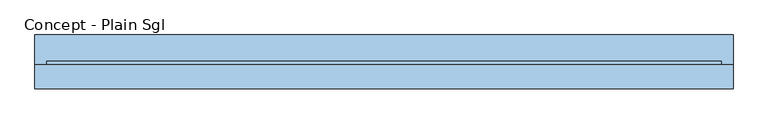
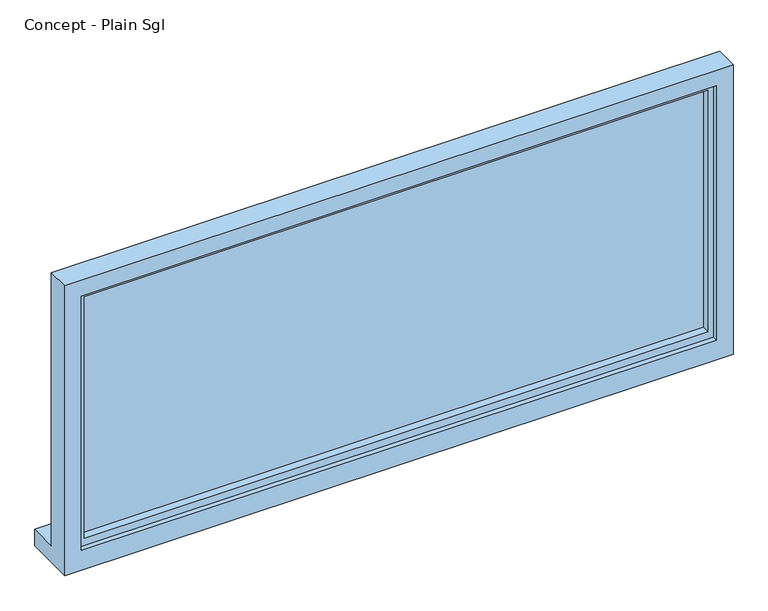
"""IFC4 building model written with IfcOpenShell, lengths in millimetres: window geometry, Concept - Plain Sgl : Visiuon Panel no Opening Sashes."""

import ifcopenshell
import ifcopenshell.guid

model = None  # the IFC model being written
_history = None  # IfcOwnerHistory: only IFC2X3 demands one
_inside = {}  # id of a spatial element -> (the spatial element, [elements in it])
_under = {}  # id of a project, library or spatial element -> (it, [spatial elements below it])
_declared = {}  # id of a project -> (the project, [libraries it declares])
_typed = {}  # id of a type object -> (the type object, [elements of that type])
_made_of = {}  # id of a material, layer set ... -> (it, [elements and type objects made of it])


def new_model(schema):
    """Start an empty IFC model of exactly this schema.

    Asked for "IFC4X3", IfcOpenShell would pick the latest addendum, in which some entities
    have other attributes; the version numbers below select the first issue.
    IFC2X3 requires an IfcOwnerHistory on every rooted entity: one is made here for all.
    """
    global model, _history
    if schema == "IFC4X3":
        model = ifcopenshell.file(schema_version=(4, 3, 0, 0))
    else:
        model = ifcopenshell.file(schema=schema)
    _inside.clear()
    _under.clear()
    _declared.clear()
    _typed.clear()
    _made_of.clear()
    _history = None
    if model.schema == "IFC2X3":
        org = make("IfcOrganization", Name="unknown")
        user = make(
            "IfcPersonAndOrganization",
            ThePerson=make("IfcPerson", FamilyName="unknown"),
            TheOrganization=org,
        )
        app = make(
            "IfcApplication",
            ApplicationDeveloper=org,
            Version="unknown",
            ApplicationFullName="unknown",
            ApplicationIdentifier="unknown",
        )
        _history = make(
            "IfcOwnerHistory",
            OwningUser=user,
            OwningApplication=app,
            ChangeAction="ADDED",
            CreationDate=0,
        )
    return model


def make(cls, **values):
    """One entity of the class cls with the attributes given. An attribute that is None is left unset."""
    return model.create_entity(
        cls, **{name: value for name, value in values.items() if value is not None}
    )


def rooted(cls, **values):
    """An entity with a GlobalId (a new one), such as an element, a storey or a relation."""
    return make(cls, GlobalId=ifcopenshell.guid.new(), OwnerHistory=_history, **values)


def si_unit(unit_type, name, prefix=None):
    """IfcSIUnit, for example si_unit("LENGTHUNIT", "METRE", prefix="MILLI")."""
    return make("IfcSIUnit", UnitType=unit_type, Prefix=prefix, Name=name)


def assignment(units):
    """IfcUnitAssignment: the units of a project."""
    return None if units is None else make("IfcUnitAssignment", Units=units)


def point(xyz):
    """IfcCartesianPoint."""
    return None if xyz is None else make("IfcCartesianPoint", Coordinates=xyz)


def direction(xyz):
    """IfcDirection."""
    return None if xyz is None else make("IfcDirection", DirectionRatios=xyz)


def frame(location, z_axis=None, x_axis=None):
    """IfcAxis2Placement3D, a coordinate frame: its origin and axes. An axis left out is left unset."""
    return make(
        "IfcAxis2Placement3D",
        Location=point(location),
        Axis=direction(z_axis),
        RefDirection=direction(x_axis),
    )


def origin():
    """The frame at (0, 0, 0) with its axes left unset."""
    return frame((0.0, 0.0, 0.0))


def place(relative_to, where):
    """IfcLocalPlacement: puts the frame where relative to a parent placement (None: the world)."""
    return make(
        "IfcLocalPlacement", PlacementRelTo=relative_to, RelativePlacement=where
    )


def context(
    kind, dimensions, precision=None, world=None, true_north=None, identifier=None
):
    """IfcGeometricRepresentationContext, for example the 3D "Model" context."""
    return make(
        "IfcGeometricRepresentationContext",
        ContextIdentifier=identifier,
        ContextType=kind,
        CoordinateSpaceDimension=dimensions,
        Precision=precision,
        WorldCoordinateSystem=world,
        TrueNorth=true_north,
    )


def project(units=None, contexts=None):
    """IfcProject with its units and contexts."""
    return rooted(
        "IfcProject",
        Name="project",
        RepresentationContexts=contexts,
        UnitsInContext=assignment(units),
    )


def spatial(cls, under=None, at=None, **own):
    """A site, building, storey or space (cls), placed at a placement, below another one or the project."""
    s = rooted(cls, ObjectPlacement=at, **own)
    if under is not None:
        _under.setdefault(under.id(), (under, []))[1].append(s)
    return s


def polyline(points):
    """IfcPolyline through the points."""
    return make("IfcPolyline", Points=[point(p) for p in points])


def outline(outer, holes=None, kind="AREA"):
    """IfcArbitraryClosedProfileDef: a profile drawn as a closed curve; with holes, ...WithVoids."""
    if holes is None:
        return make("IfcArbitraryClosedProfileDef", ProfileType=kind, OuterCurve=outer)
    return make(
        "IfcArbitraryProfileDefWithVoids",
        ProfileType=kind,
        OuterCurve=outer,
        InnerCurves=holes,
    )


def extrude(swept, where, along, depth):
    """IfcExtrudedAreaSolid: the profile swept, set in the frame where, extruded along a direction by depth."""
    return make(
        "IfcExtrudedAreaSolid",
        SweptArea=swept,
        Position=where,
        ExtrudedDirection=direction(along),
        Depth=depth,
    )


def faces_of(points, faces, orient=None, outer=None):
    """IfcFace entities. A face is a list of loops; a loop is a list of indices into points, from 0.

    orient and outer hold one flag for each loop. By default every Orientation is true, the
    first loop of a face is its IfcFaceOuterBound and the others are IfcFaceBound.
    """
    made = []
    for i, loops in enumerate(faces):
        bounds = []
        for j, loop in enumerate(loops):
            is_outer = j == 0 if outer is None else outer[i][j]
            bounds.append(
                make(
                    "IfcFaceOuterBound" if is_outer else "IfcFaceBound",
                    Bound=make("IfcPolyLoop", Polygon=[points[k] for k in loop]),
                    Orientation=True if orient is None else orient[i][j],
                )
            )
        made.append(make("IfcFace", Bounds=bounds))
    return made


def faceted_brep(points, faces, orient=None, outer=None, voids=None):
    """IfcFacetedBrep: a solid bounded by flat faces; with voids (closed shells), ...WithVoids."""
    shared = [point(p) for p in points]
    hull = make("IfcClosedShell", CfsFaces=faces_of(shared, faces, orient, outer))
    if voids is None:
        return make("IfcFacetedBrep", Outer=hull)
    return make(
        "IfcFacetedBrepWithVoids",
        Outer=hull,
        Voids=[
            make(cls, CfsFaces=faces_of(shared, fs, o, b)) for cls, fs, o, b in voids
        ],
    )


def shape(context_of_items, identifier, shape_type, items):
    """IfcShapeRepresentation: the items that make up one representation, for example the "Body"."""
    return make(
        "IfcShapeRepresentation",
        ContextOfItems=context_of_items,
        RepresentationIdentifier=identifier,
        RepresentationType=shape_type,
        Items=items,
    )


def source(mapping_origin, context_of_items, identifier, shape_type, items):
    """IfcRepresentationMap: a shape defined once, which mapped items show again and again."""
    return make(
        "IfcRepresentationMap",
        MappingOrigin=mapping_origin,
        MappedRepresentation=shape(context_of_items, identifier, shape_type, items),
    )


def transform(
    local_origin,
    x_axis=None,
    y_axis=None,
    z_axis=None,
    scale=None,
    scale2=None,
    scale3=None,
    uniform=True,
):
    """IfcCartesianTransformationOperator3D, or its non-uniform kind. x_axis, y_axis, z_axis: its Axis1, 2, 3."""
    if uniform:
        return make(
            "IfcCartesianTransformationOperator3D",
            Axis1=direction(x_axis),
            Axis2=direction(y_axis),
            LocalOrigin=point(local_origin),
            Scale=scale,
            Axis3=direction(z_axis),
        )
    return make(
        "IfcCartesianTransformationOperator3DnonUniform",
        Axis1=direction(x_axis),
        Axis2=direction(y_axis),
        LocalOrigin=point(local_origin),
        Scale=scale,
        Axis3=direction(z_axis),
        Scale2=scale2,
        Scale3=scale3,
    )


def mapped(mapping_source, mapping_target):
    """IfcMappedItem: shows the shape of a source again, moved by a transform."""
    return make(
        "IfcMappedItem", MappingSource=mapping_source, MappingTarget=mapping_target
    )


def made_of(thing, what):
    """Note that an element or type object is made of a material, layer set ...; save() writes the relation."""
    if what is not None:
        _made_of.setdefault(what.id(), (what, []))[1].append(thing)
    return thing


def element(
    cls,
    number,
    at=None,
    inside=None,
    cuts=None,
    type_object=None,
    material=None,
    context=None,
    identifier="Body",
    shape_type=None,
    held_by="IfcProductDefinitionShape",
    body=None,
    shapes=None,
    **own,
):
    """One element of the class cls, such as IfcWall. Its Tag is "e" and its number.

    at: its placement. inside: the storey or other place that contains it. cuts: it is an
    opening in that element (IfcRelVoidsElement). A single representation is given by context,
    identifier, shape_type and body (its items); several are given by shapes. held_by: the class
    of the entity that holds the representations. save() writes the other relations.
    """
    e = rooted(cls, Tag="e%d" % number, ObjectPlacement=at, **own)
    if body is not None:
        shapes = [shape(context, identifier, shape_type, body)]
    if shapes is not None:
        e.Representation = make(held_by, Representations=shapes)
    if inside is not None:
        _inside.setdefault(inside.id(), (inside, []))[1].append(e)
    if cuts is not None:
        rooted(
            "IfcRelVoidsElement", RelatingBuildingElement=cuts, RelatedOpeningElement=e
        )
    if type_object is not None:
        _typed.setdefault(type_object.id(), (type_object, []))[1].append(e)
    return made_of(e, material)


def aggregate(whole, parts):
    """IfcRelAggregates: a whole, such as a stair, and the parts it consists of."""
    return rooted("IfcRelAggregates", RelatingObject=whole, RelatedObjects=parts)


def save(model, path):
    """Write the relations noted so far, then the file.

    IfcRelAggregates (storeys below a building ...), IfcRelContainedInSpatialStructure (elements
    in a storey), IfcRelDefinesByType, IfcRelAssociatesMaterial and IfcRelDeclares: one each for
    every whole, place, type object, material and project.
    """
    for whole, parts in _under.values():
        aggregate(whole, parts)
    for where, things in _inside.values():
        rooted(
            "IfcRelContainedInSpatialStructure",
            RelatedElements=things,
            RelatingStructure=where,
        )
    for kind, things in _typed.values():
        rooted("IfcRelDefinesByType", RelatedObjects=things, RelatingType=kind)
    for what, things in _made_of.values():
        rooted("IfcRelAssociatesMaterial", RelatedObjects=things, RelatingMaterial=what)
    for by, libraries in _declared.values():
        rooted("IfcRelDeclares", RelatingContext=by, RelatedDefinitions=libraries)
    model.write(path)


def concept_plain_sgl_1110da93(model_context):
    return source(origin(), model_context, "Body", "SolidModel", [
        faceted_brep([(-1200.0, -27.0434322, 1010.0), (1200.0, -27.0434322, 1010.0), (1200.0, -27.0434322, 2110.0), (-1200.0, -27.0434322, 2110.0), (-1140.0, -27.0434322, 2050.0), (1140.0, -27.0434322, 2050.0), (1140.0, -27.0434322, 1085.0), (-1140.0, -27.0434322, 1085.0), (-1200.0, 55.9565678, 2110.0), (-1200.0, 55.9565678, 1073.0), (-1200.0, 158.4565678, 1073.0), (-1200.0, 158.4565678, 1010.0), (1200.0, 55.9565678, 2110.0), (1200.0, 55.9565678, 1073.0), (1160.0, 55.9565678, 1073.0), (1160.0, 55.9565678, 2070.0), (-1160.0, 55.9565678, 2070.0), (-1160.0, 55.9565678, 1073.0), (-1160.0, -9.0434322, 2070.0), (-1160.0, -9.0434322, 1073.0), (1160.0, -9.0434322, 2070.0), (1160.0, -9.0434322, 1073.0), (-1140.0, -9.0434322, 2050.0), (-1140.0, -9.0434322, 1085.0), (1140.0, -9.0434322, 1085.0), (1140.0, -9.0434322, 2050.0), (1200.0, 158.4565678, 1010.0), (1200.0, 158.4565678, 1073.0)], [[[0, 1, 2, 3], [4, 5, 6, 7]], [[0, 3, 8, 9, 10, 11]], [[9, 8, 12, 13, 14, 15, 16, 17]], [[17, 16, 18, 19]], [[18, 20, 21, 19], [22, 23, 24, 25]], [[22, 4, 7, 23]], [[3, 2, 12, 8]], [[16, 15, 20, 18]], [[5, 4, 22, 25]], [[13, 12, 2, 1, 26, 27]], [[15, 14, 21, 20]], [[5, 25, 24, 6]], [[26, 1, 0, 11]], [[27, 26, 11, 10]], [[27, 10, 9, 17, 19, 21, 14, 13]], [[7, 6, 24, 23]]]),
        extrude(outline(polyline([(1130.0, 19.9565678), (-1130.0, 19.9565678), (-1130.0, 43.9565678), (1130.0, 43.9565678), (1130.0, 19.9565678)])), frame((0.0, 0.0, 1103.0), z_axis=(0.0, 0.0, 1.0), x_axis=(1.0, 0.0, 0.0)), (0.0, 0.0, 1.0), 937.0),
        faceted_brep([(-1160.0, -9.0434322, 2070.0), (-1160.0, 67.5035732, 2070.0), (-1160.0, 67.5035732, 1073.0), (-1160.0, -9.0434322, 1073.0), (-1120.0, 19.9565678, 2030.0), (-1120.0, -9.0434322, 2030.0), (-1120.0, -9.0434322, 1113.0), (-1120.0, 19.9565678, 1113.0), (-1130.0, 43.9565678, 2040.0), (-1130.0, 19.9565678, 2040.0), (-1130.0, 19.9565678, 1103.0), (-1130.0, 43.9565678, 1103.0), (-1120.0, 67.5035732, 2030.0), (-1120.0, 43.9565678, 2030.0), (-1120.0, 43.9565678, 1113.0), (-1120.0, 67.5035732, 1113.0), (1160.0, 67.5035732, 1073.0), (1160.0, -9.0434322, 1073.0), (1120.0, -9.0434322, 1113.0), (1120.0, 19.9565678, 1113.0), (1130.0, 19.9565678, 1103.0), (1130.0, 43.9565678, 1103.0), (1120.0, 43.9565678, 1113.0), (1120.0, 67.5035732, 1113.0), (1160.0, 67.5035732, 2070.0), (1160.0, -9.0434322, 2070.0), (1120.0, -9.0434322, 2030.0), (1120.0, 19.9565678, 2030.0), (1130.0, 19.9565678, 2040.0), (1130.0, 43.9565678, 2040.0), (1120.0, 43.9565678, 2030.0), (1120.0, 67.5035732, 2030.0)], [[[0, 1, 2, 3]], [[4, 5, 6, 7]], [[8, 9, 10, 11]], [[12, 13, 14, 15]], [[3, 2, 16, 17]], [[7, 6, 18, 19]], [[11, 10, 20, 21]], [[15, 14, 22, 23]], [[17, 16, 24, 25]], [[19, 18, 26, 27]], [[21, 20, 28, 29]], [[23, 22, 30, 31]], [[1, 24, 16, 2], [15, 23, 31, 12]], [[25, 24, 1, 0]], [[3, 17, 25, 0], [5, 26, 18, 6]], [[27, 26, 5, 4]], [[9, 28, 20, 10], [7, 19, 27, 4]], [[29, 28, 9, 8]], [[11, 21, 29, 8], [13, 30, 22, 14]], [[31, 30, 13, 12]]]),
    ])


if __name__ == "__main__":
    model = new_model("IFC4")
    model_context = context("Model", 3, world=origin())
    ifc_project = project(units=[si_unit("LENGTHUNIT", "METRE", prefix="MILLI")], contexts=[model_context])
    site = spatial("IfcSite", under=ifc_project)
    building = spatial("IfcBuilding", under=site)
    placement = place(None, origin())
    concept_plain_sgl_shape = concept_plain_sgl_1110da93(model_context)
    element("IfcWindow", 1, ObjectType="Concept - Plain Sgl : Visiuon Panel no Opening Sashes", at=placement, inside=building, context=model_context, shape_type="MappedRepresentation", body=[
        mapped(concept_plain_sgl_shape, transform((0.0, 0.0, 0.0), x_axis=(1.0, 0.0, 0.0), y_axis=(0.0, 1.0, 0.0), z_axis=(0.0, 0.0, 1.0))),
    ])
    save(model, "model.ifc")

# Revit data of these elements
# Type "Concept - Plain Sgl : Visiuon Panel no Opening Sashes"
#   Type Mark = "44"
#   Operation = "SinglePanel"
#   Description = "Half Hour Vision Panel"
#   Manufacturer = "Revit"
#   Keynote = "L10"
#   Visual Light Transmittance = 0.9
#   Solar Heat Gain Coefficient = 0.86
#   Rough Width = 2400 mm
#   Rough Height = 1100 mm
#   Height = 1100 mm
#   Width = 2400 mm
#   Heat Transfer Coefficient (U) = 5.5617 W/(m²·K)
#   FrameOffset - External = 0 mm
#   Default Head Height = 2110 mm
#   Define Thermal Properties by = 1
#   Material Trim = Window Frame
#   Material Glass = Glass
#   Material Frame = Window Frame
#   Construction Type Id = ""
#   Wall Closure = (empty or 0)
#   Analytic Construction = (empty or 0)
# Element 1 (IfcWindow, "Concept - Plain Sgl : Visiuon Panel no Opening Sashes")
#   Materials on its faces: "Window Frame", "Glass"
# Materials
#   "Window Frame": class "Miscellaneous", colour RGB 249 249 249, transparency 0, Keynote = "L10"
#   "Glass": class "Glass", colour RGB 0 128 192, transparency 0.9, Description = "Soda Lime Glass", Cost = 0
